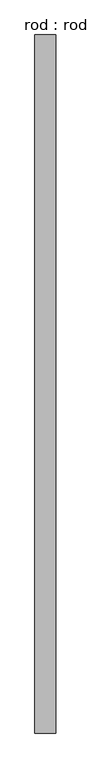
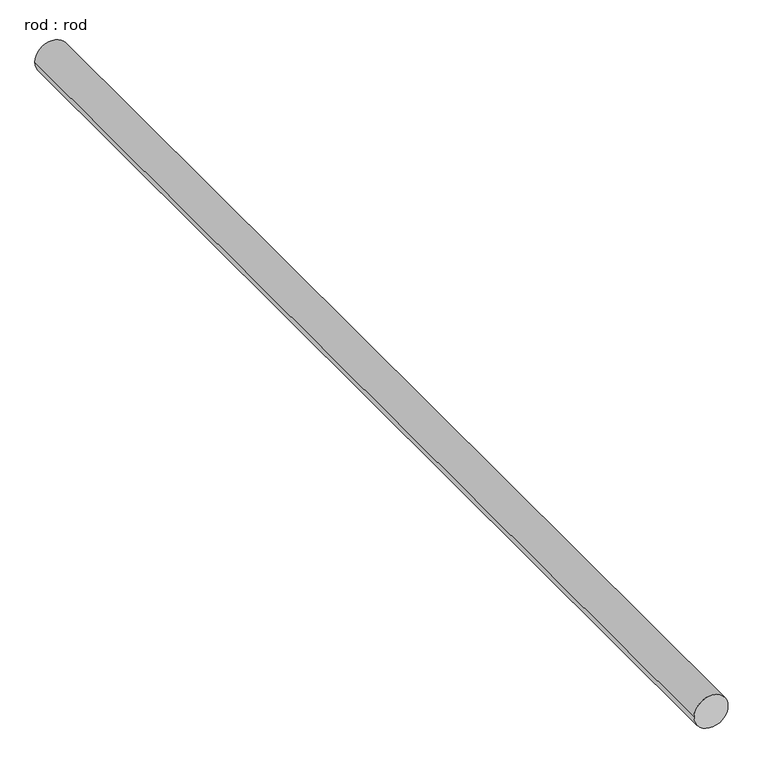
"""IFC4 building model written with IfcOpenShell, lengths in millimetres: proxy geometry, rod : rod."""

from ifc_helpers import new_model, si_unit, point, frame, frame_2d, origin, place, context, project, spatial, circle_curve, trimmed, segment, composite_curve, outline, extrude, source, transform, mapped, element, save


def rod_rod_d42026ae(model_context):
    return source(origin(), model_context, "Body", "SweptSolid", [
        extrude(outline(composite_curve([segment(trimmed(circle_curve(frame_2d((0.0108462, 0.0)), 200.0), [point((0.0108462, 200.0))], [point((0.0108462, -200.0))], False, "CARTESIAN"), True, "CONTINUOUS"), segment(trimmed(circle_curve(frame_2d((0.0108462, 0.0)), 200.0), [point((0.0108462, -200.0))], [point((0.0108462, 200.0))], False, "CARTESIAN"), True, "CONTINUOUS")], self_intersect=False)), frame((0.0, -2633.9463333, 0.0), z_axis=(0.0, 1.0, 0.0), x_axis=(0.0, 0.0, 1.0)), (0.0, 0.0, 1.0), 13453.3498972),
    ])


if __name__ == "__main__":
    model = new_model("IFC4")
    model_context = context("Model", 3, world=origin())
    ifc_project = project(units=[si_unit("LENGTHUNIT", "METRE", prefix="MILLI")], contexts=[model_context])
    site = spatial("IfcSite", under=ifc_project)
    building = spatial("IfcBuilding", under=site)
    placement = place(None, origin())
    rod_rod_shape = rod_rod_d42026ae(model_context)
    element("IfcBuildingElementProxy", 1, Name="rod : rod", ObjectType="rod : rod", at=placement, inside=building, context=model_context, shape_type="MappedRepresentation", body=[
        mapped(rod_rod_shape, transform((0.0, 0.0, 0.0), x_axis=(1.0, 0.0, 0.0), y_axis=(0.0, 1.0, 0.0), z_axis=(0.0, 0.0, 1.0))),
    ])
    save(model, "model.ifc")

# Revit data of these elements
# Type "rod : rod"
#   Default Elevation = 0
